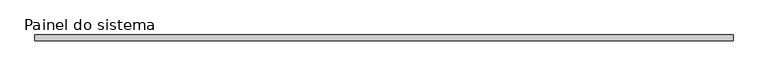
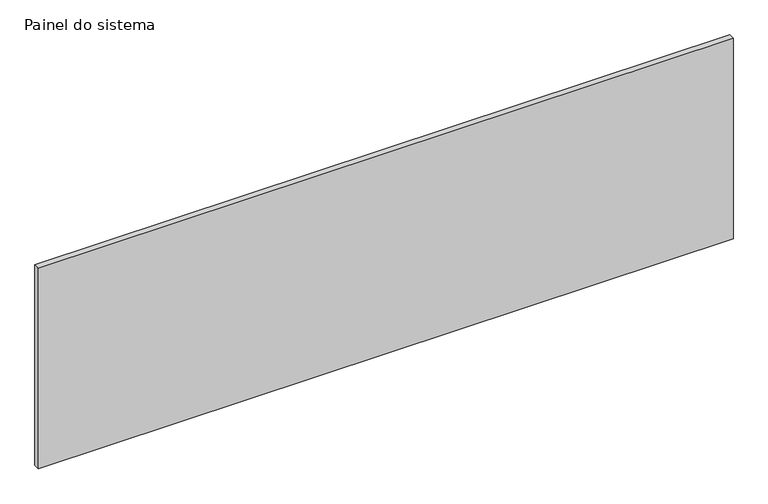
"""IFC4 building model written with IfcOpenShell, lengths in millimetres: plate geometry, Painel do sistema : Envidraçado."""

from ifc_helpers import new_model, si_unit, origin, origin_with_axes, place, context, project, spatial, polyline, outline, extrude, source, transform, mapped, element, save


def painel_do_sistema_d8fd150b(model_context):
    return source(origin(), model_context, "Body", "SweptSolid", [
        extrude(outline(polyline([(1475.0, -49.5), (-1475.0, -49.5), (-1475.0, -24.5), (1475.0, -24.5), (1475.0, -49.5)])), origin_with_axes(), (0.0, 0.0, 1.0), 900.0),
    ])


if __name__ == "__main__":
    model = new_model("IFC4")
    model_context = context("Model", 3, world=origin())
    ifc_project = project(units=[si_unit("LENGTHUNIT", "METRE", prefix="MILLI")], contexts=[model_context])
    site = spatial("IfcSite", under=ifc_project)
    building = spatial("IfcBuilding", under=site)
    placement = place(None, origin())
    painel_do_sistema_shape = painel_do_sistema_d8fd150b(model_context)
    element("IfcPlate", 1, ObjectType="Painel do sistema : Envidraçado", at=placement, inside=building, context=model_context, shape_type="MappedRepresentation", body=[
        mapped(painel_do_sistema_shape, transform((0.0, 0.0, 0.0), x_axis=(1.0, 0.0, 0.0), y_axis=(0.0, 1.0, 0.0), z_axis=(0.0, 0.0, 1.0))),
    ])
    save(model, "model.ifc")

# Revit data of these elements
# Type "Painel do sistema : Envidraçado"
#   Construction Type Id = "GSP4R"
#   Analytic Construction = "Vidraça única Pilkington 1/8 pol"
#   Visual Light Transmittance = 0.9
#   Solar Heat Gain Coefficient = 0.86
#   Heat Transfer Coefficient (U) = 6.7069 W/(m²·K)
# Element 1 (IfcPlate, "Painel do sistema : Envidraçado")
#   Materials on its faces: "Vidro"
# Materials
#   "Vidro": class "Vidro", colour RGB 0 128 192, transparency 0.9, Description = "Vidro de sílica", Cost = 0
